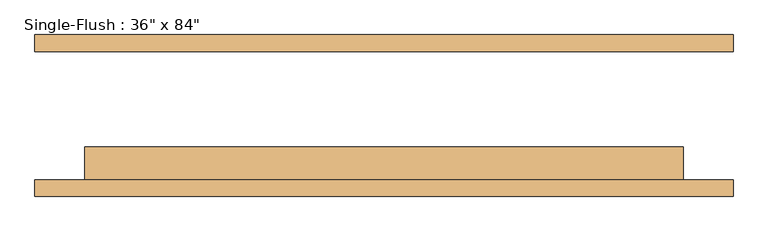
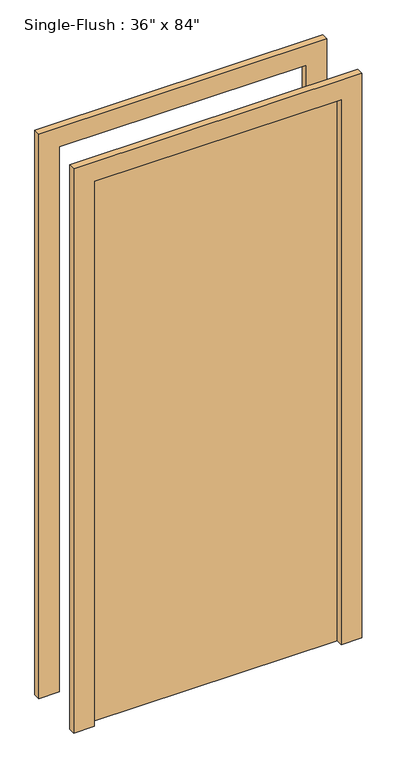
"""IFC4 building model written with IfcOpenShell, lengths in millimetres: door geometry."""

from ifc_helpers import new_model, si_unit, frame, origin, origin_with_axes, place, context, project, spatial, polyline, outline, extrude, source, transform, mapped, element, save


def door_4c327cca(model_context):
    return source(origin(), model_context, "Body", "SweptSolid", [
        extrude(outline(polyline([(2209.8, -533.4), (0.0, -533.4), (0.0, -457.2), (2133.6, -457.2), (2133.6, 457.2), (0.0, 457.2), (0.0, 533.4), (2209.8, 533.4), (2209.8, -533.4)])), frame((0.0, -123.825, 0.0), z_axis=(0.0, 1.0, 0.0), x_axis=(0.0, 0.0, 1.0)), (0.0, 0.0, 1.0), 25.4),
        extrude(outline(polyline([(2209.8, 533.4), (2209.8, -533.4), (0.0, -533.4), (0.0, -457.2), (2133.6, -457.2), (2133.6, 457.2), (0.0, 457.2), (0.0, 533.4), (2209.8, 533.4)])), frame((0.0, 98.425, 0.0), z_axis=(0.0, 1.0, 0.0), x_axis=(0.0, 0.0, 1.0)), (0.0, 0.0, 1.0), 25.4),
        extrude(outline(polyline([(457.2, -47.625), (457.2, -98.425), (-457.2, -98.425), (-457.2, -47.625), (457.2, -47.625)])), origin_with_axes(), (0.0, 0.0, 1.0), 2133.6),
    ])


if __name__ == "__main__":
    model = new_model("IFC4")
    model_context = context("Model", 3, world=origin())
    ifc_project = project(units=[si_unit("LENGTHUNIT", "METRE", prefix="MILLI")], contexts=[model_context])
    site = spatial("IfcSite", under=ifc_project)
    building = spatial("IfcBuilding", under=site)
    placement = place(None, origin())
    door_shape = door_4c327cca(model_context)
    element("IfcDoor", 1, ObjectType="Single-Flush : 36\" x 84\"", at=placement, inside=building, context=model_context, shape_type="MappedRepresentation", body=[
        mapped(door_shape, transform((0.0, 0.0, 0.0), x_axis=(1.0, 0.0, 0.0), y_axis=(0.0, 1.0, 0.0), z_axis=(0.0, 0.0, 1.0))),
    ])
    save(model, "model.ifc")

# Revit data of these elements
# Type "Single-Flush : 36\" x 84\""
#   Type Mark = "1"
#   Assembly Code = "C1020"
#   Thickness = 0' - 2"
#   Height = 7' - 0"
#   Trim Projection Ext = 0' - 1"
#   Trim Projection Int = 0' - 1"
#   Trim Width = 0' - 3"
#   Width = 3' - 0"
#   Door Material = Door - Panel
#   Frame Material = Door - Frame
#   Function = (empty or 0)
#   Wall Closure = (empty or 0)
# Element 1 (IfcDoor, "Single-Flush : 36\" x 84\"")
#   Materials on its faces: "Door - Frame", "Door - Panel"
# Materials
#   "Door - Panel": class "Wood", colour RGB 114 82 51, transparency 0
#   "Door - Frame": class "Miscellaneous", colour RGB 153 76 43, transparency 0
